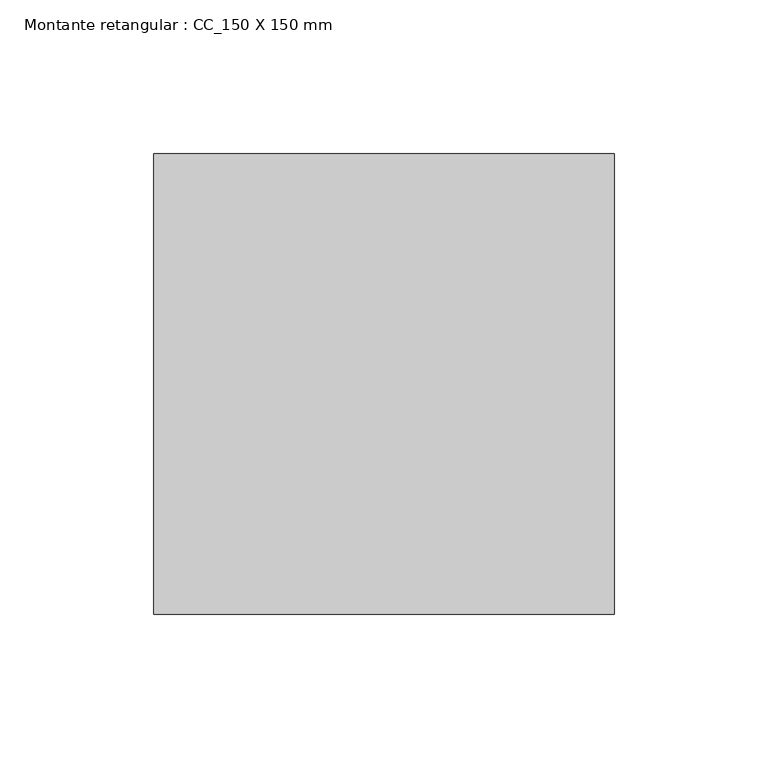
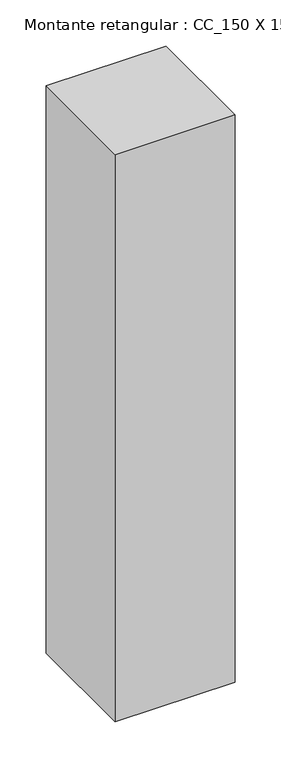
"""IFC4 building model written with IfcOpenShell, lengths in millimetres: member geometry, Montante retangular : CC_150 X 150 mm."""

from ifc_helpers import new_model, si_unit, frame, origin, place, context, project, spatial, polyline, outline, extrude, source, transform, mapped, element, save


def montante_retangular_cc_150_x_150_mm_9af7129c(model_context):
    return source(origin(), model_context, "Body", "SweptSolid", [
        extrude(outline(polyline([(0.0, 75.0), (0.0, -75.0), (-150.0, -75.0), (-150.0, 75.0), (0.0, 75.0)])), frame((0.0, 0.0, -750.0), z_axis=(0.0, 0.0, 1.0), x_axis=(1.0, 0.0, 0.0)), (0.0, 0.0, 1.0), 750.0),
    ])


if __name__ == "__main__":
    model = new_model("IFC4")
    model_context = context("Model", 3, world=origin())
    ifc_project = project(units=[si_unit("LENGTHUNIT", "METRE", prefix="MILLI")], contexts=[model_context])
    site = spatial("IfcSite", under=ifc_project)
    building = spatial("IfcBuilding", under=site)
    placement = place(None, origin())
    montante_retangular_cc_150_x_150_mm_shape = montante_retangular_cc_150_x_150_mm_9af7129c(model_context)
    element("IfcMember", 1, ObjectType="Montante retangular : CC_150 X 150 mm", at=placement, inside=building, context=model_context, shape_type="MappedRepresentation", body=[
        mapped(montante_retangular_cc_150_x_150_mm_shape, transform((0.0, 0.0, 0.0), x_axis=(1.0, 0.0, 0.0), y_axis=(0.0, 1.0, 0.0), z_axis=(0.0, 0.0, 1.0))),
    ])
    save(model, "model.ifc")

# Revit data of these elements
# Type "Montante retangular : CC_150 X 150 mm"
#   built-in parameter 1007304 = 0.492126 (stored number, unit not read)
#   built-in parameter 1007301 = 0.246063 (stored number, unit not read)
#   built-in parameter 1007300 = 0.246063 (stored number, unit not read)
# Element 1 (IfcMember, "Montante retangular : CC_150 X 150 mm")
#   Materials on its faces: ".ALUMÍNIO"
# Materials
#   ".ALUMÍNIO": class "CC_METAIS", colour RGB 244 244 244, transparency 0, Description = "Material alumínio", Cost = 0
